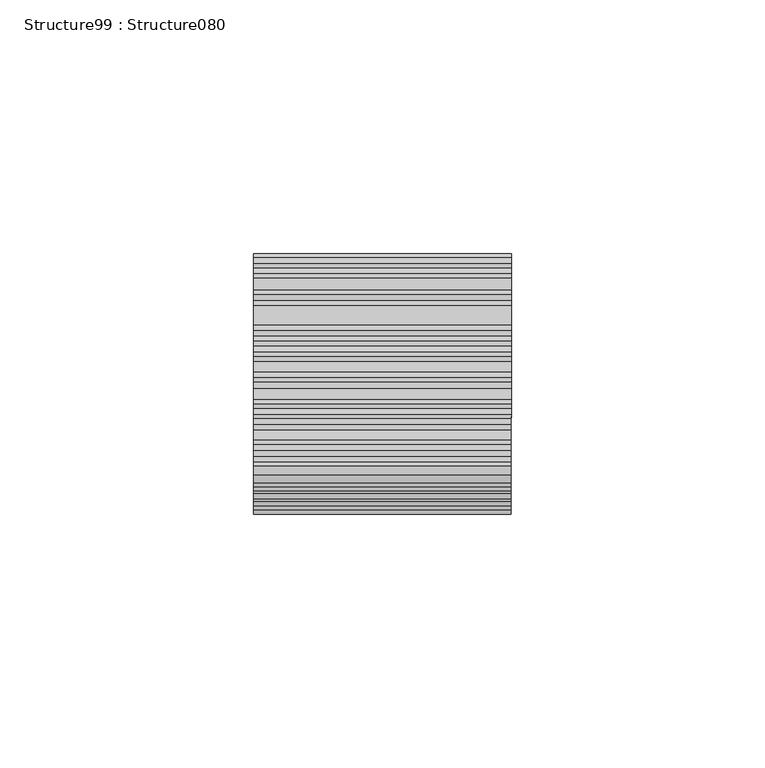
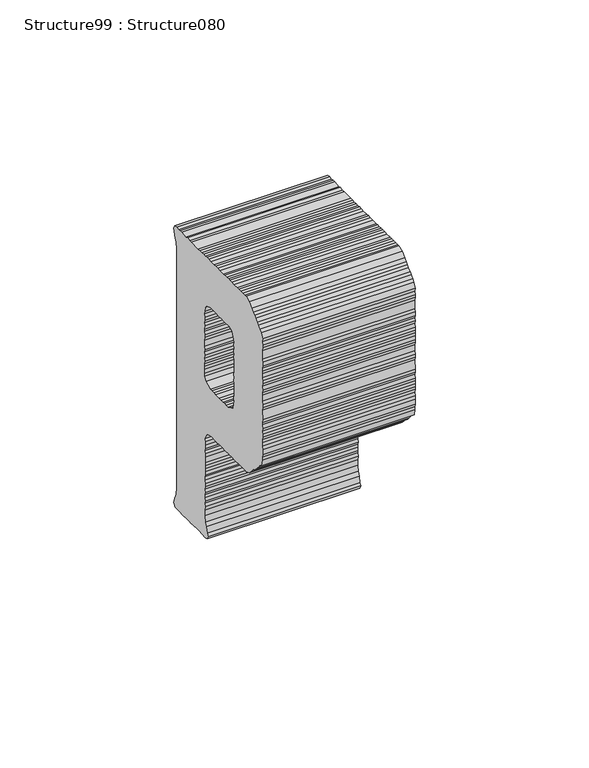
"""IFC4 building model written with IfcOpenShell, lengths in millimetres: proxy geometry, Structure99 : Structure080."""

from ifc_helpers import new_model, si_unit, frame, origin, place, context, project, spatial, polyline, outline, extrude, source, transform, mapped, element, save


def structure99_structure080_cd0925da(model_context):
    return source(origin(), model_context, "Body", "SweptSolid", [
        extrude(outline(polyline([(1.9495147, 0.0), (3.1176578, 0.256899), (4.0285462, 0.1273821), (5.3297646, 0.0), (7.407017, 0.0), (8.3161263, 0.256899), (9.2252356, 0.0), (10.396937, 0.256899), (11.1751061, 0.1273821), (12.3428934, 0.1273821), (13.5145948, 0.0), (15.4644653, 0.1273821), (16.3700164, 0.1273821), (17.5417178, 0.256899), (18.7112842, 0.1273821), (19.7499104, 0.1273821), (20.5280795, 0.256899), (22.348433, -0.5248282), (23.9061945, -1.9537844), (24.6861427, -2.8628937), (25.4660909, -3.5097668), (25.987361, -4.1623329), (27.0256314, -4.9380113), (27.5451225, -5.7240084), (28.4542318, -6.6270688), (29.2345358, -7.2796349), (30.0141281, -8.9708273), (29.7533151, -10.1368356), (30.0141281, -11.3028439), (30.0141281, -12.0884851), (29.7533151, -13.2541376), (29.7533151, -16.2447692), (30.0141281, -17.2833954), (30.0141281, -18.5824788), (29.7533151, -19.4972812), (29.8846111, -20.4006974), (29.7533151, -21.4396795), (29.8846111, -22.7441001), (30.0141281, -23.6535653), (30.0141281, -24.6864985), (29.8846111, -25.7286829), (30.0141281, -27.0277663), (29.8846111, -28.0667483), (29.7533151, -28.9797716), (29.7533151, -31.0609381), (30.0141281, -32.0931596), (30.0141281, -33.264861), (29.7533151, -34.307757), (30.0141281, -37.425059), (29.8846111, -38.5932022), (29.7533151, -39.3731504), (30.0141281, -40.6722338), (29.8846111, -41.5777849), (30.0141281, -42.6199693), (30.0141281, -43.6585956), (29.8846111, -44.5680607), (29.7533151, -45.7376272), (29.8846111, -46.9096843), (30.0141281, -47.9479548), (30.0141281, -49.7665292), (29.7533151, -50.8090694), (29.7533151, -51.8455608), (29.365476, -53.9228132), (28.3250707, -54.4458624), (27.8055796, -55.2218966), (26.2478181, -57.0401153), (25.595252, -57.6926814), (24.5587607, -58.2121724), (23.2575423, -59.7681548), (22.348433, -60.8103392), (20.5280795, -61.4589914), (19.7499104, -61.3298302), (18.5821231, -61.1963993), (16.3700164, -61.1963993), (15.3331693, -61.4589914), (14.2927639, -61.3298302), (13.2523585, -61.4589914), (12.4741895, -61.3298302), (11.1751061, -61.3298302), (10.2659968, -61.1963993), (9.0960745, -61.4589914), (8.3161263, -61.3298302), (7.0188221, -61.1963993), (5.0671724, -61.1963993), (3.8972502, -61.4589914), (2.98992, -61.3298302), (2.0808107, -61.3298302), (1.0404054, -61.1963993), (-0.2590338, -61.4589914), (-1.9498704, -61.9763475), (-2.4672266, -62.6289136), (-3.2471748, -64.320106), (-2.9863617, -65.2292153), (-3.1176577, -66.5243847), (-2.9863617, -67.566925), (-3.2471748, -68.4760343), (-2.9863617, -69.3854994), (-3.1176577, -70.6845828), (-3.1176577, -72.6362323), (-2.9863617, -73.6748586), (-3.1176577, -74.7134848), (-3.1176577, -75.7499762), (-2.9863617, -76.9216775), (-3.2471748, -77.7016257), (-3.2471748, -78.8694131), (-2.9863617, -79.9062602), (-3.1176577, -81.0818755), (-3.2471748, -81.9870709), (-2.9863617, -83.1587722), (-3.2471748, -83.9387204), (-3.2471748, -84.9773466), (-3.1176577, -86.270737), (-3.2471748, -87.0563782), (-2.9863617, -88.0950045), (-3.2471748, -89.3940879), (-3.2471748, -91.3421792), (-2.9863617, -93.4229899), (-2.3380655, -94.7163802), (-1.9498704, -96.7975467), (-1.4286003, -97.579274), (-1.9498704, -98.6157653), (-2.9863617, -98.8783574), (-5.1966894, -98.8783574), (-6.3648326, -98.7491962), (-7.2739419, -98.6157653), (-10.3915996, -98.8783574), (-11.3028438, -98.8783574), (-12.3414701, -98.7491962), (-13.2523585, -98.8783574), (-14.2909847, -98.7491962), (-15.459128, -98.8783574), (-16.4995333, -98.8783574), (-17.2794815, -98.7491962), (-19.4876741, -98.7491962), (-20.3971393, -98.8783574), (-21.1749526, -97.579274), (-20.9184094, -96.7975467), (-20.5263004, -95.7606995), (-20.0089443, -94.4594812), (-19.8776483, -93.6798889), (-19.4876741, -91.3421792), (-19.4876741, -90.4327141), (-19.6171911, -89.2667058), (-19.6171911, -88.3519035), (-19.358513, -87.3150563), (-19.6171911, -86.1472689), (-19.6171911, -85.2342456), (-19.358513, -84.3286945), (-19.358513, -83.2865101), (-19.4876741, -81.9870709), (-19.4876741, -81.0818755), (-19.358513, -80.0393353), (-19.4876741, -79.130226), (-19.6171911, -78.0876858), (-19.358513, -76.7886024), (-19.6171911, -75.8830513), (-19.6171911, -74.970028), (-19.4876741, -73.9314017), (-19.4876741, -72.6362323), (-19.6171911, -71.723209), (-19.4876741, -70.5572007), (-19.358513, -69.5185745), (-19.4876741, -68.7386263), (-19.4876741, -67.7000001), (-19.358513, -66.3952236), (-19.358513, -64.4474881), (-19.4876741, -63.5380229), (-19.6171911, -62.3684565), (-19.4876741, -61.1963993), (-19.358513, -59.1212817), (-19.6171911, -58.2121724), (-19.4876741, -57.0401153), (-19.6171911, -56.136699), (-19.6171911, -54.0558883), (-19.4876741, -53.1407302), (-19.4876741, -51.9747219), (-19.358513, -50.9364514), (-19.6171911, -49.8939112), (-19.358513, -48.8570641), (-19.6171911, -47.9479548), (-19.358513, -46.6470923), (-19.6171911, -45.6102451), (-19.4876741, -44.8285179), (-19.358513, -43.5294345), (-19.358513, -41.5777849), (-19.6171911, -40.6722338), (-19.4876741, -39.3731504), (-19.358513, -38.3302544), (-19.358513, -37.2919839), (-19.4876741, -36.2551368), (-19.4876741, -32.2265905), (-19.358513, -31.3135673), (-19.6171911, -30.1457799), (-19.4876741, -29.2363148), (-19.6171911, -27.9372314), (-19.358513, -26.90074), (-19.4876741, -25.9916307), (-19.358513, -25.0803865), (-19.358513, -21.7001367), (-19.4876741, -20.6632895), (-19.4876741, -19.8812064), (-19.358513, -18.71164), (-19.6171911, -17.5438526), (-19.4876741, -16.6343875), (-19.4876741, -14.4258389), (-19.6171911, -13.5170855), (-19.6171911, -11.4362748), (-19.358513, -10.5268097), (-19.6171911, -9.2334193), (-19.358513, -7.4091519), (-19.8776483, -5.0714422), (-20.2658433, -4.032816), (-20.5263004, -2.9959688), (-20.9184094, -2.2142415), (-21.3062486, -1.0443193), (-20.5263004, 0.1273821), (-19.358513, 0.256899), (-18.4490479, 0.0), (-17.4086426, 0.256899), (-16.4995333, 0.256899), (-14.1618236, 0.0), (-13.2523585, 0.256899), (-12.0806571, 0.0), (-11.0441658, 0.1273821), (-7.2739419, 0.0), (-6.1061545, 0.1273821), (-5.0675282, 0.0), (-4.0271229, 0.1273821), (-3.1176577, 0.0), (-1.9498704, 0.256899), (-1.0386262, 0.256899), (0.0, 0.0), (1.9495147, 0.0)]), holes=[polyline([(-2.5985226, -43.6585956), (0.0, -44.8285179), (0.9108884, -44.9580348), (2.0808107, -44.8285179), (3.1176578, -44.9580348), (5.0671724, -45.085061), (6.2388739, -44.9580348), (7.275721, -45.085061), (8.0556692, -44.9580348), (9.0960745, -45.085061), (10.2659968, -44.9580348), (11.8237583, -44.1816448), (12.7350025, -43.7916707), (13.1228416, -41.9734521), (13.3832987, -41.1917248), (13.1228416, -39.8926414), (13.3832987, -38.8536594), (13.3832987, -37.8168122), (13.2523585, -36.7728487), (13.3832987, -35.7360015), (13.2523585, -34.8211992), (13.1228416, -33.784352), (13.3832987, -32.7460816), (13.1228416, -31.5743802), (13.3832987, -30.7979902), (13.2523585, -29.7558058), (13.2523585, -28.8463407), (13.3832987, -27.8094935), (13.3832987, -26.6377922), (13.1228416, -25.5995217), (13.3832987, -24.4331576), (13.1228416, -23.6535653), (13.2523585, -22.4818639), (13.1228416, -21.3101626), (13.2523585, -20.4006974), (13.1228416, -19.3645619), (12.4741895, -17.9356058), (12.0863503, -17.1538785), (10.396937, -16.5016682), (8.3161263, -16.5016682), (7.0188221, -16.6343875), (6.1075779, -16.3739303), (4.9380113, -16.6343875), (4.1580632, -16.5016682), (3.1176578, -16.3739303), (-0.1295169, -16.3739303), (-2.0772524, -17.0264964), (-2.7276837, -17.8060888), (-3.1176577, -19.3645619), (-3.2471748, -20.4006974), (-3.1176577, -21.4396795), (-3.1176577, -22.6152948), (-3.3763359, -23.6535653), (-3.1176577, -24.4331576), (-3.2471748, -25.7286829), (-3.3763359, -26.6377922), (-3.1176577, -27.6806882), (-3.1176577, -28.5897975), (-3.2471748, -29.6223749), (-3.2471748, -31.7031855), (-3.1176577, -32.8791567), (-3.2471748, -33.6555467), (-3.1176577, -34.8211992), (-3.2471748, -35.9989494), (-3.1176577, -36.9023656), (-3.3763359, -38.0680181), (-3.2471748, -38.8536594), (-3.3763359, -39.8926414), (-3.2471748, -41.1917248), (-3.2471748, -42.2299952), (-2.5985226, -43.6585956)])]), frame((-56111.1232903, 292121.6268111, -276.7221981), z_axis=(-0.9999998917542983, 0.0004652863545059615, 0.0), x_axis=(-0.0004652863545059615, -0.9999998917542983, 0.0)), (0.0, 0.0, 1.0), 50.8),
    ])


if __name__ == "__main__":
    model = new_model("IFC4")
    model_context = context("Model", 3, world=origin())
    ifc_project = project(units=[si_unit("LENGTHUNIT", "METRE", prefix="MILLI")], contexts=[model_context])
    site = spatial("IfcSite", under=ifc_project)
    building = spatial("IfcBuilding", under=site)
    placement = place(None, origin())
    structure99_structure080_shape = structure99_structure080_cd0925da(model_context)
    element("IfcBuildingElementProxy", 1, Name="Structure99 : Structure080", ObjectType="Structure99 : Structure080", at=placement, inside=building, context=model_context, shape_type="MappedRepresentation", body=[
        mapped(structure99_structure080_shape, transform((0.0, 0.0, 0.0), x_axis=(1.0, 0.0, 0.0), y_axis=(0.0, 1.0, 0.0), z_axis=(0.0, 0.0, 1.0))),
    ])
    save(model, "model.ifc")

# Revit data of these elements
# Type "Structure99 : Structure080"
#   NameOverride = "Structure080"
# Element 1 (IfcBuildingElementProxy, "Structure99 : Structure080")
#   Materials on its faces: "BRUSHED ALUMINUM LETTERING"
# Materials
#   "BRUSHED ALUMINUM LETTERING": class "Unassigned", colour RGB 169 181 186, transparency 0, Cost = 0
